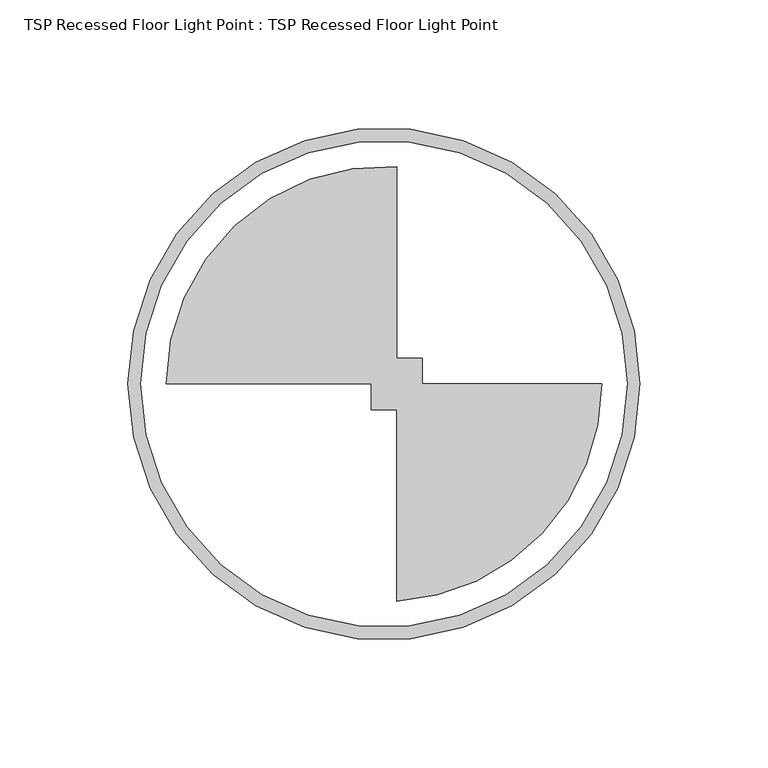
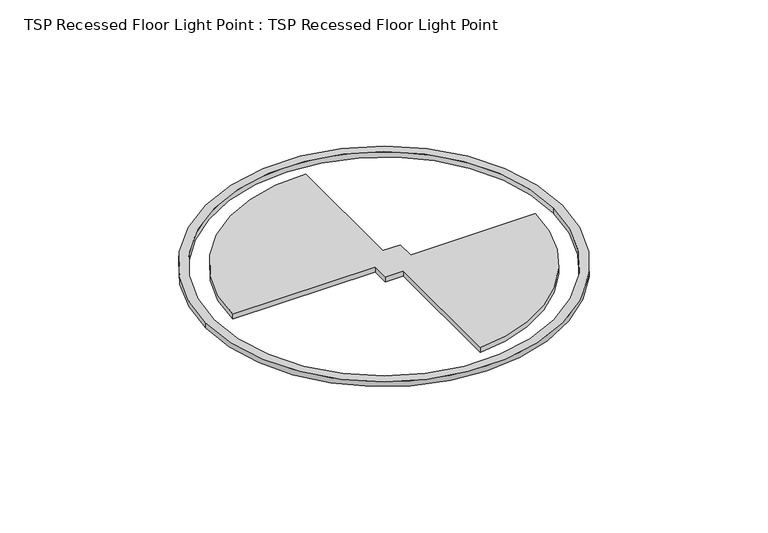
"""IFC4 building model written with IfcOpenShell, lengths in millimetres: proxy geometry, TSP Recessed Floor Light Point : TSP Recessed Floor Light Point."""

from ifc_helpers import new_model, si_unit, point, frame_2d, origin, origin_with_axes, place, context, project, spatial, polyline, circle_curve, trimmed, segment, composite_curve, outline, extrude, source, transform, mapped, element, save


def tsp_recessed_floor_light_point_tsp_recessed_floor_light_ca54e027(model_context):
    return source(origin(), model_context, "Body", "SweptSolid", [
        extrude(outline(composite_curve([segment(trimmed(circle_curve(frame_2d((-5.0, 0.0)), 100.0), [point((-105.0, 0.0))], [point((95.0, 0.0))], False, "CARTESIAN"), True, "CONTINUOUS"), segment(trimmed(circle_curve(frame_2d((-5.0, 0.0)), 100.0), [point((95.0, 0.0))], [point((-105.0, 0.0))], False, "CARTESIAN"), True, "CONTINUOUS")], self_intersect=False), holes=[composite_curve([segment(trimmed(circle_curve(frame_2d((-5.0, 0.0)), 95.0), [point((-100.0, 0.0))], [point((90.0, 0.0))], True, "CARTESIAN"), True, "CONTINUOUS"), segment(trimmed(circle_curve(frame_2d((-5.0, 0.0)), 95.0), [point((90.0, 0.0))], [point((-100.0, 0.0))], True, "CARTESIAN"), True, "CONTINUOUS")], self_intersect=False)]), origin_with_axes(), (0.0, 0.0, 1.0), 3.0),
        extrude(outline(composite_curve([segment(trimmed(circle_curve(frame_2d((-5.0, 0.0)), 85.0), [point((-90.0, 0.0))], [point((0.0, 84.8528137))], False, "CARTESIAN"), True, "CONTINUOUS"), segment(polyline([(0.0, 84.8528137), (0.0, 10.0), (10.0, 10.0), (10.0, 0.0), (80.0, 0.0)]), True, "CONTINUOUS"), segment(trimmed(circle_curve(frame_2d((-5.0, 0.0)), 85.0), [point((80.0, 0.0))], [point((0.0, -84.8528137))], False, "CARTESIAN"), True, "CONTINUOUS"), segment(polyline([(0.0, -84.8528137), (0.0, -10.0), (-10.0, -10.0), (-10.0, 0.0), (-90.0, 0.0)]), True, "CONTINUOUS")], self_intersect=False)), origin_with_axes(), (0.0, 0.0, 1.0), 3.0),
    ])


if __name__ == "__main__":
    model = new_model("IFC4")
    model_context = context("Model", 3, world=origin())
    ifc_project = project(units=[si_unit("LENGTHUNIT", "METRE", prefix="MILLI")], contexts=[model_context])
    site = spatial("IfcSite", under=ifc_project)
    building = spatial("IfcBuilding", under=site)
    placement = place(None, origin())
    tsp_recessed_floor_light_point_tsp_recessed_floor_light_shape = tsp_recessed_floor_light_point_tsp_recessed_floor_light_ca54e027(model_context)
    element("IfcBuildingElementProxy", 1, Name="TSP Recessed Floor Light Point : TSP Recessed Floor Light Point", ObjectType="TSP Recessed Floor Light Point : TSP Recessed Floor Light Point", at=placement, inside=building, context=model_context, shape_type="MappedRepresentation", body=[
        mapped(tsp_recessed_floor_light_point_tsp_recessed_floor_light_shape, transform((0.0, 0.0, 0.0), x_axis=(1.0, 0.0, 0.0), y_axis=(0.0, 1.0, 0.0), z_axis=(0.0, 0.0, 1.0))),
    ])
    save(model, "model.ifc")

# Revit data of these elements
# Type "TSP Recessed Floor Light Point : TSP Recessed Floor Light Point"
#   Model = "TSP_ELEC220RFLP"
#   Default Elevation = 0
# Element 1 (IfcBuildingElementProxy, "TSP Recessed Floor Light Point : TSP Recessed Floor Light Point")
#   Materials on its faces: "Plastic, Opaque Black"
# Materials
#   "Plastic, Opaque Black": class "Plastic", colour RGB 0 0 0, transparency 0.7, Description = "Plastic, generic, opaque black", Cost = 0
